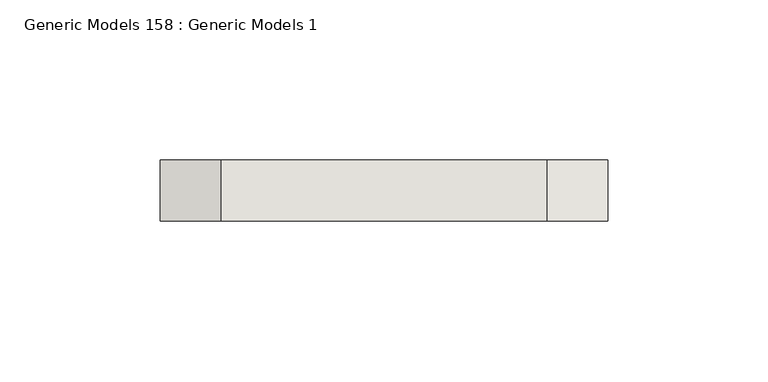
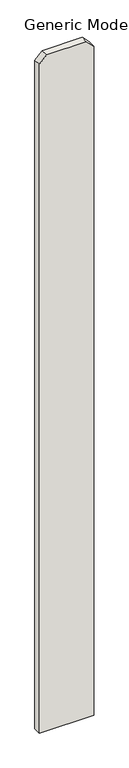
"""IFC4 building model written with IfcOpenShell, lengths in millimetres: wall geometry, Generic Models 158 : Generic Models 1."""

from ifc_helpers import new_model, si_unit, frame, origin, place, context, project, spatial, polyline, outline, extrude, source, transform, mapped, element, save


def generic_models_158_generic_models_1_4322e38f(model_context):
    return source(origin(), model_context, "Body", "SweptSolid", [
        extrude(outline(polyline([(76.2, 323061.0125), (1885.95, 323061.0125), (1905.0, 323041.9625), (1905.0, 322940.3625), (1885.95, 322921.3125), (76.2, 322921.3125), (76.2, 323061.0125)])), frame((0.0, 547.6875, 0.0), z_axis=(0.0, 1.0, 0.0), x_axis=(0.0, 0.0, 1.0)), (0.0, 0.0, 1.0), 19.05),
    ])


if __name__ == "__main__":
    model = new_model("IFC4")
    model_context = context("Model", 3, world=origin())
    ifc_project = project(units=[si_unit("LENGTHUNIT", "METRE", prefix="MILLI")], contexts=[model_context])
    site = spatial("IfcSite", under=ifc_project)
    building = spatial("IfcBuilding", under=site)
    placement = place(None, origin())
    generic_models_158_generic_models_1_shape = generic_models_158_generic_models_1_4322e38f(model_context)
    element("IfcWall", 1, ObjectType="Generic Models 158 : Generic Models 1", at=placement, inside=building, context=model_context, shape_type="MappedRepresentation", body=[
        mapped(generic_models_158_generic_models_1_shape, transform((0.0, 0.0, 0.0), x_axis=(1.0, 0.0, 0.0), y_axis=(0.0, 1.0, 0.0), z_axis=(0.0, 0.0, 1.0))),
    ])
    save(model, "model.ifc")

# Revit data of these elements
# Element 1 (IfcWall, "Generic Models 158 : Generic Models 1")
#   Materials on its faces: "VERTICAL 1X6 CEDAR PLANKS W/ CLEAR WOOD SEALER"
# Materials
#   "VERTICAL 1X6 CEDAR PLANKS W/ CLEAR WOOD SEALER": class "Wood", colour RGB 234 198 147, transparency 0, Description = "Pinus Echinata", Cost = 0
